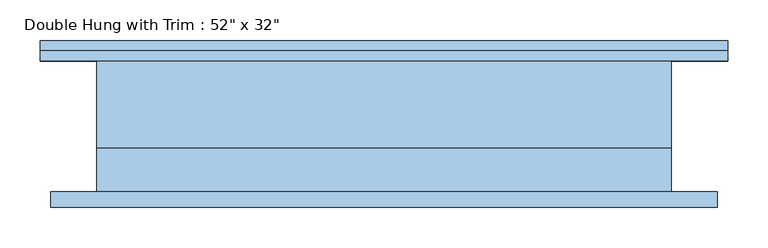
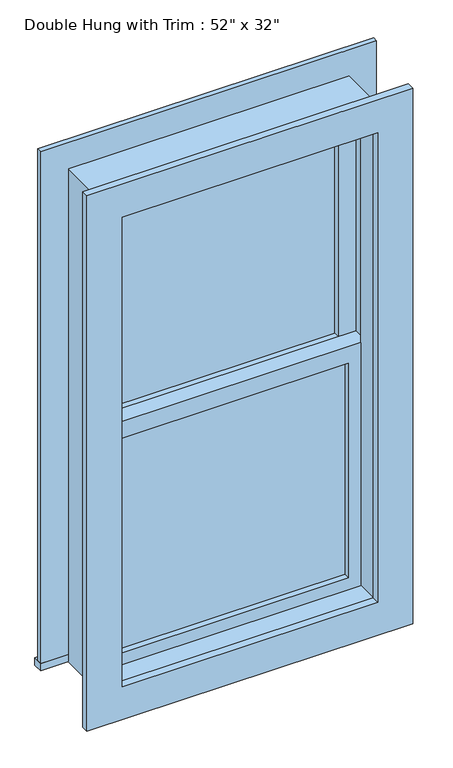
"""IFC4 building model written with IfcOpenShell, lengths in millimetres: window geometry."""

from ifc_helpers import new_model, si_unit, frame, origin, place, context, project, spatial, polyline, outline, extrude, source, transform, mapped, element, save


def window_979bf23a(model_context):
    return source(origin(), model_context, "Body", "SweptSolid", [
        extrude(outline(polyline([(-292.1, 1.5875), (292.1, 1.5875), (292.1, -11.1125), (-292.1, -11.1125), (-292.1, 1.5875)])), frame((0.0, 0.0, 977.9), z_axis=(0.0, 0.0, 1.0), x_axis=(1.0, 0.0, 0.0)), (0.0, 0.0, 1.0), 574.675),
        extrude(outline(polyline([(1597.025, -336.55), (933.45, -336.55), (933.45, 336.55), (1597.025, 336.55), (1597.025, -336.55)]), holes=[polyline([(1552.575, -292.1), (1552.575, 292.1), (977.9, 292.1), (977.9, -292.1), (1552.575, -292.1)])]), frame((0.0, -26.9875, 0.0), z_axis=(0.0, 1.0, 0.0), x_axis=(0.0, 0.0, 1.0)), (0.0, 0.0, 1.0), 44.45),
        extrude(outline(polyline([(-425.45, 106.3625), (425.45, 106.3625), (425.45, 80.9625), (-425.45, 80.9625), (-425.45, 106.3625)])), frame((0.0, 0.0, 914.4), z_axis=(0.0, 0.0, 1.0), x_axis=(1.0, 0.0, 0.0)), (0.0, 0.0, 1.0), 19.05),
        extrude(outline(polyline([(2216.15, -336.55), (2216.15, 336.55), (933.45, 336.55), (933.45, 425.45), (2305.05, 425.45), (2305.05, -425.45), (933.45, -425.45), (933.45, -336.55), (2216.15, -336.55)])), frame((0.0, 80.9625, 0.0), z_axis=(0.0, 1.0, 0.0), x_axis=(0.0, 0.0, 1.0)), (0.0, 0.0, 1.0), 12.7),
        extrude(outline(polyline([(2292.35, 412.75), (2292.35, -412.75), (857.25, -412.75), (857.25, 412.75), (2292.35, 412.75)]), holes=[polyline([(2203.45, 323.85), (946.15, 323.85), (946.15, -323.85), (2203.45, -323.85), (2203.45, 323.85)])]), frame((0.0, -100.0125, 0.0), z_axis=(0.0, 1.0, 0.0), x_axis=(0.0, 0.0, 1.0)), (0.0, 0.0, 1.0), 19.05),
        extrude(outline(polyline([(292.1, 33.3375), (-292.1, 33.3375), (-292.1, 46.0375), (292.1, 46.0375), (292.1, 33.3375)])), frame((0.0, 0.0, 1597.025), z_axis=(0.0, 0.0, 1.0), x_axis=(1.0, 0.0, 0.0)), (0.0, 0.0, 1.0), 574.675),
        extrude(outline(polyline([(2216.15, -336.55), (1552.575, -336.55), (1552.575, 336.55), (2216.15, 336.55), (2216.15, -336.55)]), holes=[polyline([(2171.7, -292.1), (2171.7, 292.1), (1597.025, 292.1), (1597.025, -292.1), (2171.7, -292.1)])]), frame((0.0, 17.4625, 0.0), z_axis=(0.0, 1.0, 0.0), x_axis=(0.0, 0.0, 1.0)), (0.0, 0.0, 1.0), 44.45),
        extrude(outline(polyline([(2235.2, -355.6), (914.4, -355.6), (914.4, 355.6), (2235.2, 355.6), (2235.2, -355.6)]), holes=[polyline([(2203.45, -323.85), (2203.45, 323.85), (946.15, 323.85), (946.15, -323.85), (2203.45, -323.85)])]), frame((0.0, -80.9625, 0.0), z_axis=(0.0, 1.0, 0.0), x_axis=(0.0, 0.0, 1.0)), (0.0, 0.0, 1.0), 53.975),
        extrude(outline(polyline([(2235.2, 355.6), (2235.2, -355.6), (914.4, -355.6), (914.4, 355.6), (2235.2, 355.6)]), holes=[polyline([(2216.15, 336.55), (933.45, 336.55), (933.45, -336.55), (2216.15, -336.55), (2216.15, 336.55)])]), frame((0.0, -26.9875, 0.0), z_axis=(0.0, 1.0, 0.0), x_axis=(0.0, 0.0, 1.0)), (0.0, 0.0, 1.0), 107.95),
    ])


if __name__ == "__main__":
    model = new_model("IFC4")
    model_context = context("Model", 3, world=origin())
    ifc_project = project(units=[si_unit("LENGTHUNIT", "METRE", prefix="MILLI")], contexts=[model_context])
    site = spatial("IfcSite", under=ifc_project)
    building = spatial("IfcBuilding", under=site)
    placement = place(None, origin())
    window_shape = window_979bf23a(model_context)
    element("IfcWindow", 1, ObjectType="Double Hung with Trim : 52\" x 32\"", at=placement, inside=building, context=model_context, shape_type="MappedRepresentation", body=[
        mapped(window_shape, transform((0.0, 0.0, 0.0), x_axis=(1.0, 0.0, 0.0), y_axis=(0.0, 1.0, 0.0), z_axis=(0.0, 0.0, 1.0))),
    ])
    save(model, "model.ifc")

# Revit data of these elements
# Type "Double Hung with Trim : 52\" x 32\""
#   Type Mark = "61"
#   COBie.Type.CreatedBy = "doug.wood@us.ibm.com"
#   COBie.Type.CreatedOn = "2016-04-14T02:07:26"
#   COBie.Type.Name = "Windows_Double Hung with Trim_52\" x 32\"_61"
#   COBie.Type.Category = "23-30 20 17 17 14 : Double-Hung Windows"
#   COBie.Type.Description = "Double Hung with Trim_52\" x 32\""
#   COBie.Type.Manufacturer = ""
#   COBie.Type.ModelNumber = ""
#   Construction Type Id = "GSP4R"
#   Assembly Code = "B2020100"
#   Analytic Construction = "1/8 in Pilkington single glazing"
#   COBie.Type.ReplacementCost = 0
#   Visual Light Transmittance = 0.9
#   Solar Heat Gain Coefficient = 0.78
#   Heat Transfer Coefficient (U) = 3.6886 W/(m²·K)
#   Height = 4' - 4"
#   Default Sill Height = 3' - 0"
#   Trim Projection - Ext. = 0' - 0 1/2"
#   Trim Projection - Int. = 0' - 0 3/4"
#   Trim Width - Exterior = 0' - 3 1/2"
#   Trim Width - Interior = 0' - 3 1/2"
#   Width = 2' - 4"
#   Window Inset = 0' - 0 3/4"
#   COBie.Type = no
#   Glass Pane Material = Glass
#   Sash Material = Sash - White
#   Trim Exterior Material = Trim - White
#   Trim Interior Material = Trim - White
#   Wall Closure = (empty or 0)
# Element 1 (IfcWindow, "Double Hung with Trim : 52\" x 32\"")
#   Materials on its faces: "Sash - White", "Trim - White", "Glass"
# Materials
#   "Glass": class "Glass", colour RGB 0 128 192, transparency 0.75, Description = "Soda Lime Glass", Cost = 0
#   "Sash - White": class "Wood", colour RGB 255 255 255, transparency 0, Cost = 0
#   "Trim - White": class "Wood", colour RGB 255 255 255, transparency 0, Cost = 0
